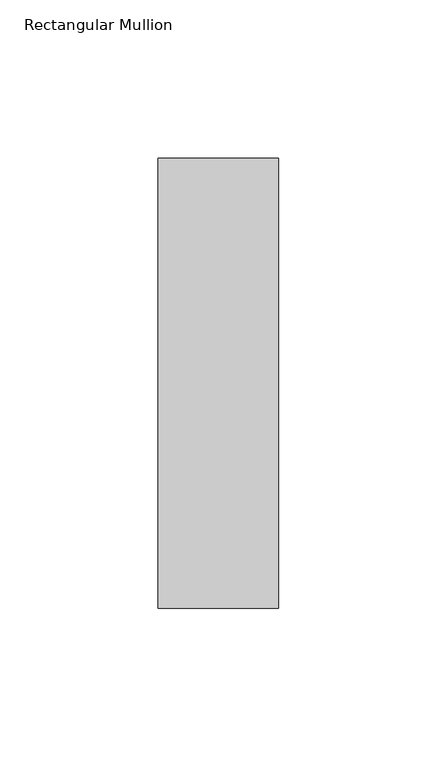
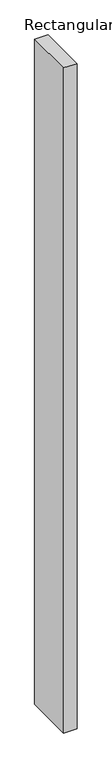
"""IFC4 building model written with IfcOpenShell, lengths in millimetres: member geometry, Rectangular Mullion : NLRS_21_CWM_hsb-regel 38x142_gen_rsf."""

from ifc_helpers import new_model, si_unit, frame, origin, place, context, project, spatial, polyline, outline, extrude, source, transform, mapped, element, save


def rectangular_mullion_39ed0f6f(model_context):
    return source(origin(), model_context, "Body", "SweptSolid", [
        extrude(outline(polyline([(-38.0, -71.0), (-38.0, 71.0), (0.0, 71.0), (0.0, -71.0), (-38.0, -71.0)])), frame((0.0, 0.0, -2000.0), z_axis=(0.0, 0.0, 1.0), x_axis=(1.0, 0.0, 0.0)), (0.0, 0.0, 1.0), 2000.0),
    ])


if __name__ == "__main__":
    model = new_model("IFC4")
    model_context = context("Model", 3, world=origin())
    ifc_project = project(units=[si_unit("LENGTHUNIT", "METRE", prefix="MILLI")], contexts=[model_context])
    site = spatial("IfcSite", under=ifc_project)
    building = spatial("IfcBuilding", under=site)
    placement = place(None, origin())
    rectangular_mullion_shape = rectangular_mullion_39ed0f6f(model_context)
    element("IfcMember", 1, ObjectType="Rectangular Mullion : NLRS_21_CWM_hsb-regel 38x142_gen_rsf", at=placement, inside=building, context=model_context, shape_type="MappedRepresentation", body=[
        mapped(rectangular_mullion_shape, transform((0.0, 0.0, 0.0), x_axis=(1.0, 0.0, 0.0), y_axis=(0.0, 1.0, 0.0), z_axis=(0.0, 0.0, 1.0))),
    ])
    save(model, "model.ifc")

# Revit data of these elements
# Type "Rectangular Mullion : NLRS_21_CWM_hsb-regel 38x142_gen_rsf"
#   Export Type to IFC As = "IfcWall"
#   Type IfcGUID = "07M7mRoiH1CR8m_RSKIwpF"
#   Assembly Code = "21.10"
#   built-in parameter 1007322 = 0.465879 (stored number, unit not read)
#   built-in parameter 1007321 = 0.062336 (stored number, unit not read)
#   built-in parameter 1007320 = 0.062336 (stored number, unit not read)
# Element 1 (IfcMember, "Rectangular Mullion : NLRS_21_CWM_hsb-regel 38x142_gen_rsf")
#   Materials on its faces: "NLRS_i2_hout naaldhout vuren_gen_rsf"
# Materials
#   "NLRS_i2_hout naaldhout vuren_gen_rsf": class "I - Hout", colour RGB 234 199 147, transparency 0, Keynote = "i2", Manufacturer = "Revit Standards Foundation", URL = "www.revitstandards.org", Description = "hout vuren", Cost = 0
